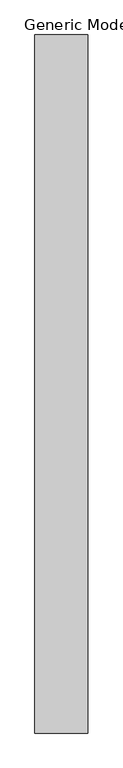
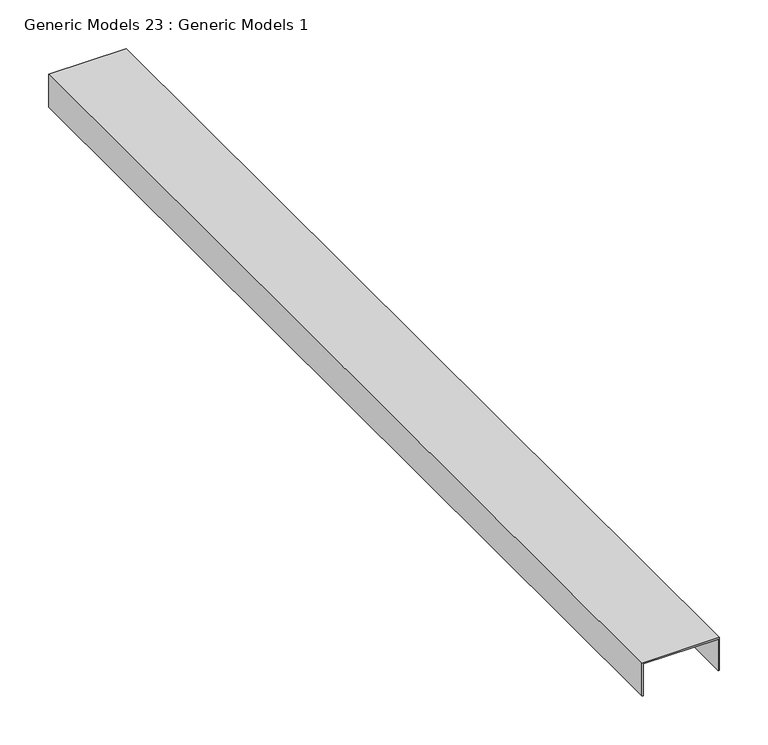
"""IFC4 building model written with IfcOpenShell, lengths in millimetres: proxy geometry, Generic Models 23 : Generic Models 1."""

import ifcopenshell
import ifcopenshell.guid

model = None  # the IFC model being written
_history = None  # IfcOwnerHistory: only IFC2X3 demands one
_inside = {}  # id of a spatial element -> (the spatial element, [elements in it])
_under = {}  # id of a project, library or spatial element -> (it, [spatial elements below it])
_declared = {}  # id of a project -> (the project, [libraries it declares])
_typed = {}  # id of a type object -> (the type object, [elements of that type])
_made_of = {}  # id of a material, layer set ... -> (it, [elements and type objects made of it])


def new_model(schema):
    """Start an empty IFC model of exactly this schema.

    Asked for "IFC4X3", IfcOpenShell would pick the latest addendum, in which some entities
    have other attributes; the version numbers below select the first issue.
    IFC2X3 requires an IfcOwnerHistory on every rooted entity: one is made here for all.
    """
    global model, _history
    if schema == "IFC4X3":
        model = ifcopenshell.file(schema_version=(4, 3, 0, 0))
    else:
        model = ifcopenshell.file(schema=schema)
    _inside.clear()
    _under.clear()
    _declared.clear()
    _typed.clear()
    _made_of.clear()
    _history = None
    if model.schema == "IFC2X3":
        org = make("IfcOrganization", Name="unknown")
        user = make(
            "IfcPersonAndOrganization",
            ThePerson=make("IfcPerson", FamilyName="unknown"),
            TheOrganization=org,
        )
        app = make(
            "IfcApplication",
            ApplicationDeveloper=org,
            Version="unknown",
            ApplicationFullName="unknown",
            ApplicationIdentifier="unknown",
        )
        _history = make(
            "IfcOwnerHistory",
            OwningUser=user,
            OwningApplication=app,
            ChangeAction="ADDED",
            CreationDate=0,
        )
    return model


def make(cls, **values):
    """One entity of the class cls with the attributes given. An attribute that is None is left unset."""
    return model.create_entity(
        cls, **{name: value for name, value in values.items() if value is not None}
    )


def rooted(cls, **values):
    """An entity with a GlobalId (a new one), such as an element, a storey or a relation."""
    return make(cls, GlobalId=ifcopenshell.guid.new(), OwnerHistory=_history, **values)


def si_unit(unit_type, name, prefix=None):
    """IfcSIUnit, for example si_unit("LENGTHUNIT", "METRE", prefix="MILLI")."""
    return make("IfcSIUnit", UnitType=unit_type, Prefix=prefix, Name=name)


def assignment(units):
    """IfcUnitAssignment: the units of a project."""
    return None if units is None else make("IfcUnitAssignment", Units=units)


def point(xyz):
    """IfcCartesianPoint."""
    return None if xyz is None else make("IfcCartesianPoint", Coordinates=xyz)


def direction(xyz):
    """IfcDirection."""
    return None if xyz is None else make("IfcDirection", DirectionRatios=xyz)


def frame(location, z_axis=None, x_axis=None):
    """IfcAxis2Placement3D, a coordinate frame: its origin and axes. An axis left out is left unset."""
    return make(
        "IfcAxis2Placement3D",
        Location=point(location),
        Axis=direction(z_axis),
        RefDirection=direction(x_axis),
    )


def origin():
    """The frame at (0, 0, 0) with its axes left unset."""
    return frame((0.0, 0.0, 0.0))


def place(relative_to, where):
    """IfcLocalPlacement: puts the frame where relative to a parent placement (None: the world)."""
    return make(
        "IfcLocalPlacement", PlacementRelTo=relative_to, RelativePlacement=where
    )


def context(
    kind, dimensions, precision=None, world=None, true_north=None, identifier=None
):
    """IfcGeometricRepresentationContext, for example the 3D "Model" context."""
    return make(
        "IfcGeometricRepresentationContext",
        ContextIdentifier=identifier,
        ContextType=kind,
        CoordinateSpaceDimension=dimensions,
        Precision=precision,
        WorldCoordinateSystem=world,
        TrueNorth=true_north,
    )


def project(units=None, contexts=None):
    """IfcProject with its units and contexts."""
    return rooted(
        "IfcProject",
        Name="project",
        RepresentationContexts=contexts,
        UnitsInContext=assignment(units),
    )


def spatial(cls, under=None, at=None, **own):
    """A site, building, storey or space (cls), placed at a placement, below another one or the project."""
    s = rooted(cls, ObjectPlacement=at, **own)
    if under is not None:
        _under.setdefault(under.id(), (under, []))[1].append(s)
    return s


def polyline(points):
    """IfcPolyline through the points."""
    return make("IfcPolyline", Points=[point(p) for p in points])


def outline(outer, holes=None, kind="AREA"):
    """IfcArbitraryClosedProfileDef: a profile drawn as a closed curve; with holes, ...WithVoids."""
    if holes is None:
        return make("IfcArbitraryClosedProfileDef", ProfileType=kind, OuterCurve=outer)
    return make(
        "IfcArbitraryProfileDefWithVoids",
        ProfileType=kind,
        OuterCurve=outer,
        InnerCurves=holes,
    )


def extrude(swept, where, along, depth):
    """IfcExtrudedAreaSolid: the profile swept, set in the frame where, extruded along a direction by depth."""
    return make(
        "IfcExtrudedAreaSolid",
        SweptArea=swept,
        Position=where,
        ExtrudedDirection=direction(along),
        Depth=depth,
    )


def shape(context_of_items, identifier, shape_type, items):
    """IfcShapeRepresentation: the items that make up one representation, for example the "Body"."""
    return make(
        "IfcShapeRepresentation",
        ContextOfItems=context_of_items,
        RepresentationIdentifier=identifier,
        RepresentationType=shape_type,
        Items=items,
    )


def source(mapping_origin, context_of_items, identifier, shape_type, items):
    """IfcRepresentationMap: a shape defined once, which mapped items show again and again."""
    return make(
        "IfcRepresentationMap",
        MappingOrigin=mapping_origin,
        MappedRepresentation=shape(context_of_items, identifier, shape_type, items),
    )


def transform(
    local_origin,
    x_axis=None,
    y_axis=None,
    z_axis=None,
    scale=None,
    scale2=None,
    scale3=None,
    uniform=True,
):
    """IfcCartesianTransformationOperator3D, or its non-uniform kind. x_axis, y_axis, z_axis: its Axis1, 2, 3."""
    if uniform:
        return make(
            "IfcCartesianTransformationOperator3D",
            Axis1=direction(x_axis),
            Axis2=direction(y_axis),
            LocalOrigin=point(local_origin),
            Scale=scale,
            Axis3=direction(z_axis),
        )
    return make(
        "IfcCartesianTransformationOperator3DnonUniform",
        Axis1=direction(x_axis),
        Axis2=direction(y_axis),
        LocalOrigin=point(local_origin),
        Scale=scale,
        Axis3=direction(z_axis),
        Scale2=scale2,
        Scale3=scale3,
    )


def mapped(mapping_source, mapping_target):
    """IfcMappedItem: shows the shape of a source again, moved by a transform."""
    return make(
        "IfcMappedItem", MappingSource=mapping_source, MappingTarget=mapping_target
    )


def made_of(thing, what):
    """Note that an element or type object is made of a material, layer set ...; save() writes the relation."""
    if what is not None:
        _made_of.setdefault(what.id(), (what, []))[1].append(thing)
    return thing


def element(
    cls,
    number,
    at=None,
    inside=None,
    cuts=None,
    type_object=None,
    material=None,
    context=None,
    identifier="Body",
    shape_type=None,
    held_by="IfcProductDefinitionShape",
    body=None,
    shapes=None,
    **own,
):
    """One element of the class cls, such as IfcWall. Its Tag is "e" and its number.

    at: its placement. inside: the storey or other place that contains it. cuts: it is an
    opening in that element (IfcRelVoidsElement). A single representation is given by context,
    identifier, shape_type and body (its items); several are given by shapes. held_by: the class
    of the entity that holds the representations. save() writes the other relations.
    """
    e = rooted(cls, Tag="e%d" % number, ObjectPlacement=at, **own)
    if body is not None:
        shapes = [shape(context, identifier, shape_type, body)]
    if shapes is not None:
        e.Representation = make(held_by, Representations=shapes)
    if inside is not None:
        _inside.setdefault(inside.id(), (inside, []))[1].append(e)
    if cuts is not None:
        rooted(
            "IfcRelVoidsElement", RelatingBuildingElement=cuts, RelatedOpeningElement=e
        )
    if type_object is not None:
        _typed.setdefault(type_object.id(), (type_object, []))[1].append(e)
    return made_of(e, material)


def aggregate(whole, parts):
    """IfcRelAggregates: a whole, such as a stair, and the parts it consists of."""
    return rooted("IfcRelAggregates", RelatingObject=whole, RelatedObjects=parts)


def save(model, path):
    """Write the relations noted so far, then the file.

    IfcRelAggregates (storeys below a building ...), IfcRelContainedInSpatialStructure (elements
    in a storey), IfcRelDefinesByType, IfcRelAssociatesMaterial and IfcRelDeclares: one each for
    every whole, place, type object, material and project.
    """
    for whole, parts in _under.values():
        aggregate(whole, parts)
    for where, things in _inside.values():
        rooted(
            "IfcRelContainedInSpatialStructure",
            RelatedElements=things,
            RelatingStructure=where,
        )
    for kind, things in _typed.values():
        rooted("IfcRelDefinesByType", RelatedObjects=things, RelatingType=kind)
    for what, things in _made_of.values():
        rooted("IfcRelAssociatesMaterial", RelatedObjects=things, RelatingMaterial=what)
    for by, libraries in _declared.values():
        rooted("IfcRelDeclares", RelatingContext=by, RelatedDefinitions=libraries)
    model.write(path)


def generic_models_23_generic_models_1_d2f1e0fb(model_context):
    return source(origin(), model_context, "Body", "SweptSolid", [
        extrude(outline(polyline([(2457.45, 49784.0), (2457.45, 49691.925), (2416.175, 49691.925), (2416.175, 49693.5125), (2455.8625, 49693.5125), (2455.8625, 49782.4125), (2416.175, 49782.4125), (2416.175, 49784.0), (2457.45, 49784.0)])), frame((0.0, 0.0, 0.0), z_axis=(0.0, 1.0, 0.0), x_axis=(0.0, 0.0, 1.0)), (0.0, 0.0, 1.0), 1219.2),
    ])


if __name__ == "__main__":
    model = new_model("IFC4")
    model_context = context("Model", 3, world=origin())
    ifc_project = project(units=[si_unit("LENGTHUNIT", "METRE", prefix="MILLI")], contexts=[model_context])
    site = spatial("IfcSite", under=ifc_project)
    building = spatial("IfcBuilding", under=site)
    placement = place(None, origin())
    generic_models_23_generic_models_1_shape = generic_models_23_generic_models_1_d2f1e0fb(model_context)
    element("IfcBuildingElementProxy", 1, Name="Generic Models 23 : Generic Models 1", ObjectType="Generic Models 23 : Generic Models 1", at=placement, inside=building, context=model_context, shape_type="MappedRepresentation", body=[
        mapped(generic_models_23_generic_models_1_shape, transform((0.0, 0.0, 0.0), x_axis=(1.0, 0.0, 0.0), y_axis=(0.0, 1.0, 0.0), z_axis=(0.0, 0.0, 1.0))),
    ])
    save(model, "model.ifc")

# Revit data of these elements
# Element 1 (IfcBuildingElementProxy, "Generic Models 23 : Generic Models 1")
#   Materials on its faces: "MATCH DEPTH OF EXISTING DEFLECTION TRACK"
# Materials
#   "MATCH DEPTH OF EXISTING DEFLECTION TRACK": class "Unassigned", colour RGB 210 209 208, transparency 0, Keynote = "M05121300.02", Cost = 0
